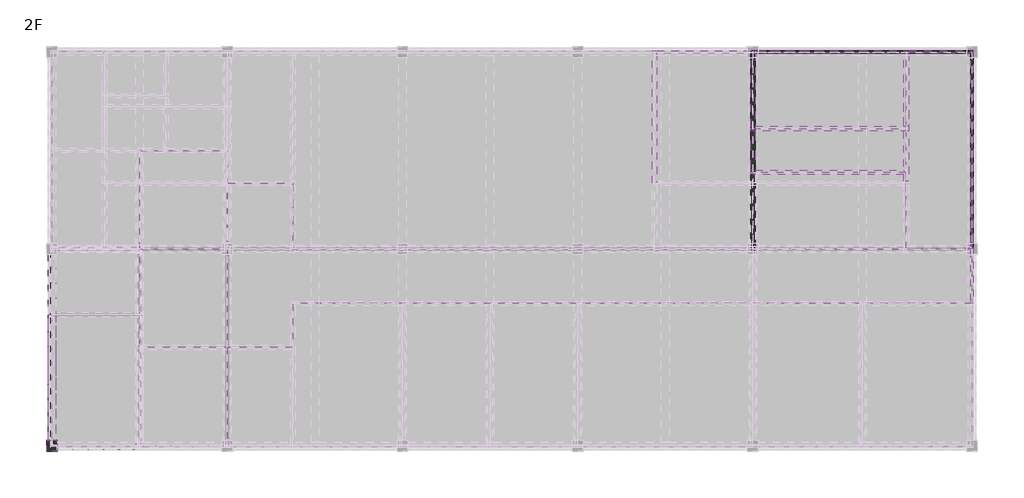
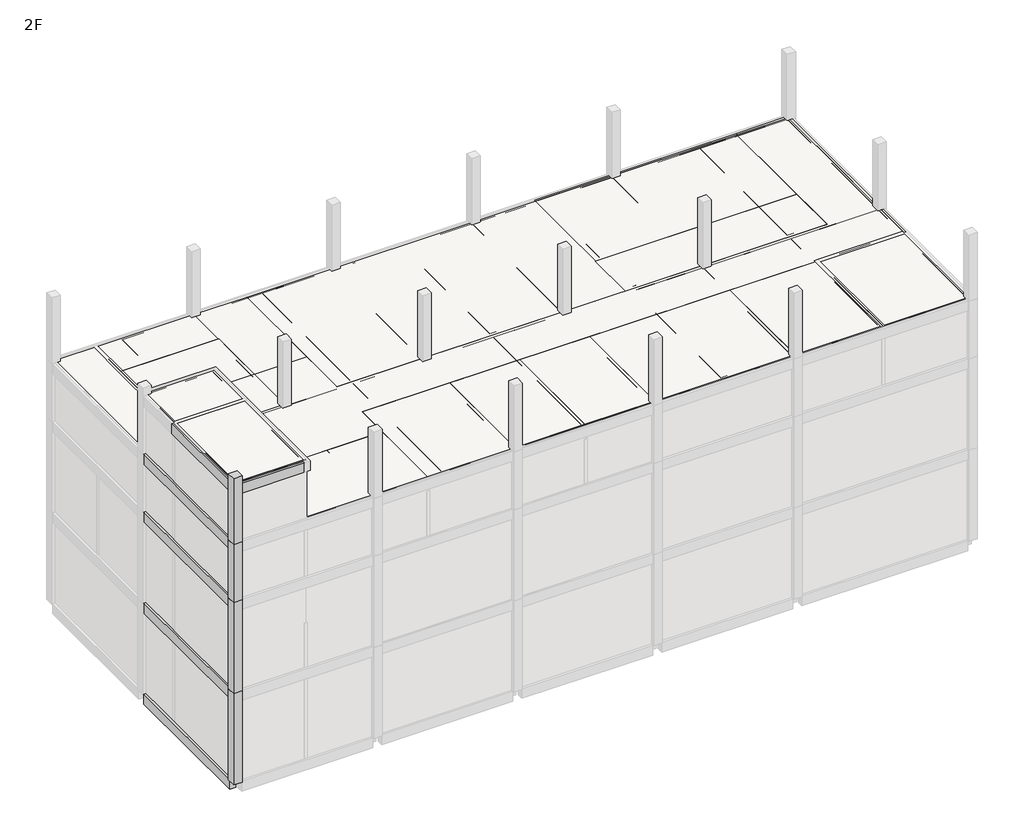
# One storey, part 3 of 7: 58 slabs, 16 walls, 6 beams, 4 columns.
# Revit data of these elements (continued)
# Materials (continued)
#   "A04AS164-00001_Plastering_Ext": class "Concrete", colour RGB 183 186 184, transparency 0, W00) Work Master Code = "A04AS164-00001", W01) Work Master_Lv1 = "Finishing Work", W02) Work Master_Lv2 = "Plastering Work", W03) Work Master_Spec.1 = "Plastering", W04) Work Master_Spec.2 = "for External Masonry Wall", Cost = 0
#   "A04AK073-00001_Concrete Brick_0.5B": class "Concrete", colour RGB 180 180 180, transparency 0, Description = "Conc. Block", W00) Work Master Code = "A04AK073-00001", W01) Work Master_Lv1 = "Finishing Work", W02) Work Master_Lv2 = "Masonry Work", W03) Work Master_Spec.1 = "Concrete Brick", W04) Work Master_Spec.2 = "[0.5B] w/ All Reinf.(Lath, Steel Tie, Anchor Bar, Mortar, ETC.), Filler, Sealant, Lintel/Sill for Opening, ETC.", Cost = 0
#   "A04AS164-00002_Plastering_Int": class "Concrete", colour RGB 183 186 184, transparency 0, Description = "LATEX PAINT ON THK.15 CEMENT PLASTER", W00) Work Master Code = "A04AS164-00002", W01) Work Master_Lv1 = "Finishing Work", W02) Work Master_Lv2 = "Plastering Work", W03) Work Master_Spec.1 = "Plastering", W04) Work Master_Spec.2 = "for Internal Masonry Wall", Cost = 0
#   "A04AL078-00002_Int Wall Painting_Water Emulsion Paint": class "Finish", colour RGB 128 128 64, transparency 0, Description = "Plastic", W00) Work Master Code = "A04AL078-00002", W01) Work Master_Lv1 = "Finishing Work", W02) Work Master_Lv2 = "Painting Work", W03) Work Master_Spec.1 = "Internal Wall Painting", W04) Work Master_Spec.2 = "Water Emulsion Paint", Cost = 0
#   "A04AK069-00002_Reinforced Concrete Block_THK 100-200mm": class "Concrete", colour RGB 180 180 180, transparency 0, Description = "Conc. Block", W00) Work Master Code = "A04AK069-00002", W01) Work Master_Lv1 = "Finishing Work", W02) Work Master_Lv2 = "Masonry Work", W03) Work Master_Spec.1 = "Reinforced Concrete Block", W04) Work Master_Spec.2 = "w/ All Reinf.(Lath, Steel Tie, Anchor Bar, Mortar, ETC.), Filler, Sealant, Lintel/Sill for Opening, ETC.", W05) Work Master_Spec.3 = "100mm<THK≤200mm", Cost = 0
#   "Default Wall": class "Miscellaneous", colour RGB 80 80 80, transparency 0
